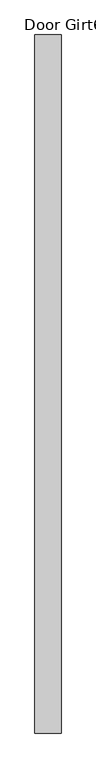
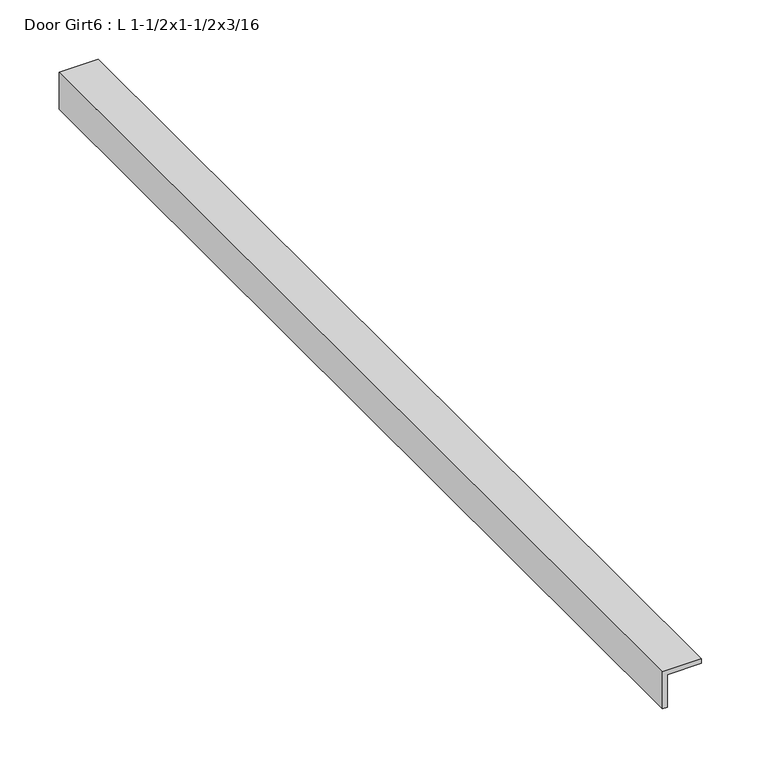
"""IFC4 building model written with IfcOpenShell, lengths in millimetres: proxy geometry, Door Girt6 : L 1-1/2x1-1/2x3/16."""

from ifc_helpers import new_model, si_unit, frame, origin, place, context, project, spatial, polyline, outline, extrude, source, transform, mapped, element, save


def door_girt6_l_1_1_2x1_1_2x3_16_599efec9(model_context):
    return source(origin(), model_context, "Body", "SweptSolid", [
        extrude(outline(polyline([(812.8, 587403.9934739), (812.8, 587365.8934739), (774.7, 587365.8934739), (774.7, 587370.6559739), (808.0375, 587370.6559739), (808.0375, 587403.9934739), (812.8, 587403.9934739)])), frame((0.0, -532839.3663841, 0.0), z_axis=(0.0, 1.0, 0.0), x_axis=(0.0, 0.0, 1.0)), (0.0, 0.0, 1.0), 1017.5875),
    ])


if __name__ == "__main__":
    model = new_model("IFC4")
    model_context = context("Model", 3, world=origin())
    ifc_project = project(units=[si_unit("LENGTHUNIT", "METRE", prefix="MILLI")], contexts=[model_context])
    site = spatial("IfcSite", under=ifc_project)
    building = spatial("IfcBuilding", under=site)
    placement = place(None, origin())
    door_girt6_l_1_1_2x1_1_2x3_16_shape = door_girt6_l_1_1_2x1_1_2x3_16_599efec9(model_context)
    element("IfcBuildingElementProxy", 1, Name="Door Girt6 : L 1-1/2x1-1/2x3/16", ObjectType="Door Girt6 : L 1-1/2x1-1/2x3/16", at=placement, inside=building, context=model_context, shape_type="MappedRepresentation", body=[
        mapped(door_girt6_l_1_1_2x1_1_2x3_16_shape, transform((0.0, 0.0, 0.0), x_axis=(1.0, 0.0, 0.0), y_axis=(0.0, 1.0, 0.0), z_axis=(0.0, 0.0, 1.0))),
    ])
    save(model, "model.ifc")

# Revit data of these elements
# Element 1 (IfcBuildingElementProxy, "Door Girt6 : L 1-1/2x1-1/2x3/16")
#   Materials on its faces: "1-1/2\"X1-1/2\" GALV. STL L"
# Materials
#   "1-1/2\"X1-1/2\" GALV. STL L": class "Generic", colour RGB 211 211 207, transparency 0, Cost = 0
